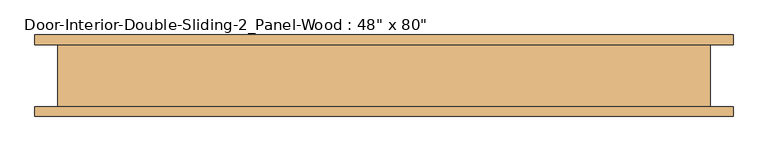
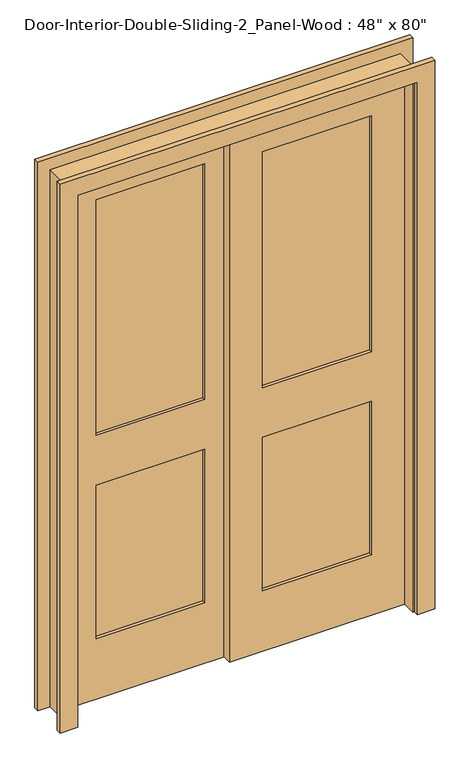
"""IFC4 building model written with IfcOpenShell, lengths in millimetres: door geometry."""

import ifcopenshell
import ifcopenshell.guid

model = None  # the IFC model being written
_history = None  # IfcOwnerHistory: only IFC2X3 demands one
_inside = {}  # id of a spatial element -> (the spatial element, [elements in it])
_under = {}  # id of a project, library or spatial element -> (it, [spatial elements below it])
_declared = {}  # id of a project -> (the project, [libraries it declares])
_typed = {}  # id of a type object -> (the type object, [elements of that type])
_made_of = {}  # id of a material, layer set ... -> (it, [elements and type objects made of it])


def new_model(schema):
    """Start an empty IFC model of exactly this schema.

    Asked for "IFC4X3", IfcOpenShell would pick the latest addendum, in which some entities
    have other attributes; the version numbers below select the first issue.
    IFC2X3 requires an IfcOwnerHistory on every rooted entity: one is made here for all.
    """
    global model, _history
    if schema == "IFC4X3":
        model = ifcopenshell.file(schema_version=(4, 3, 0, 0))
    else:
        model = ifcopenshell.file(schema=schema)
    _inside.clear()
    _under.clear()
    _declared.clear()
    _typed.clear()
    _made_of.clear()
    _history = None
    if model.schema == "IFC2X3":
        org = make("IfcOrganization", Name="unknown")
        user = make(
            "IfcPersonAndOrganization",
            ThePerson=make("IfcPerson", FamilyName="unknown"),
            TheOrganization=org,
        )
        app = make(
            "IfcApplication",
            ApplicationDeveloper=org,
            Version="unknown",
            ApplicationFullName="unknown",
            ApplicationIdentifier="unknown",
        )
        _history = make(
            "IfcOwnerHistory",
            OwningUser=user,
            OwningApplication=app,
            ChangeAction="ADDED",
            CreationDate=0,
        )
    return model


def make(cls, **values):
    """One entity of the class cls with the attributes given. An attribute that is None is left unset."""
    return model.create_entity(
        cls, **{name: value for name, value in values.items() if value is not None}
    )


def rooted(cls, **values):
    """An entity with a GlobalId (a new one), such as an element, a storey or a relation."""
    return make(cls, GlobalId=ifcopenshell.guid.new(), OwnerHistory=_history, **values)


def si_unit(unit_type, name, prefix=None):
    """IfcSIUnit, for example si_unit("LENGTHUNIT", "METRE", prefix="MILLI")."""
    return make("IfcSIUnit", UnitType=unit_type, Prefix=prefix, Name=name)


def assignment(units):
    """IfcUnitAssignment: the units of a project."""
    return None if units is None else make("IfcUnitAssignment", Units=units)


def point(xyz):
    """IfcCartesianPoint."""
    return None if xyz is None else make("IfcCartesianPoint", Coordinates=xyz)


def direction(xyz):
    """IfcDirection."""
    return None if xyz is None else make("IfcDirection", DirectionRatios=xyz)


def frame(location, z_axis=None, x_axis=None):
    """IfcAxis2Placement3D, a coordinate frame: its origin and axes. An axis left out is left unset."""
    return make(
        "IfcAxis2Placement3D",
        Location=point(location),
        Axis=direction(z_axis),
        RefDirection=direction(x_axis),
    )


def origin():
    """The frame at (0, 0, 0) with its axes left unset."""
    return frame((0.0, 0.0, 0.0))


def place(relative_to, where):
    """IfcLocalPlacement: puts the frame where relative to a parent placement (None: the world)."""
    return make(
        "IfcLocalPlacement", PlacementRelTo=relative_to, RelativePlacement=where
    )


def context(
    kind, dimensions, precision=None, world=None, true_north=None, identifier=None
):
    """IfcGeometricRepresentationContext, for example the 3D "Model" context."""
    return make(
        "IfcGeometricRepresentationContext",
        ContextIdentifier=identifier,
        ContextType=kind,
        CoordinateSpaceDimension=dimensions,
        Precision=precision,
        WorldCoordinateSystem=world,
        TrueNorth=true_north,
    )


def project(units=None, contexts=None):
    """IfcProject with its units and contexts."""
    return rooted(
        "IfcProject",
        Name="project",
        RepresentationContexts=contexts,
        UnitsInContext=assignment(units),
    )


def spatial(cls, under=None, at=None, **own):
    """A site, building, storey or space (cls), placed at a placement, below another one or the project."""
    s = rooted(cls, ObjectPlacement=at, **own)
    if under is not None:
        _under.setdefault(under.id(), (under, []))[1].append(s)
    return s


def polyline(points):
    """IfcPolyline through the points."""
    return make("IfcPolyline", Points=[point(p) for p in points])


def outline(outer, holes=None, kind="AREA"):
    """IfcArbitraryClosedProfileDef: a profile drawn as a closed curve; with holes, ...WithVoids."""
    if holes is None:
        return make("IfcArbitraryClosedProfileDef", ProfileType=kind, OuterCurve=outer)
    return make(
        "IfcArbitraryProfileDefWithVoids",
        ProfileType=kind,
        OuterCurve=outer,
        InnerCurves=holes,
    )


def extrude(swept, where, along, depth):
    """IfcExtrudedAreaSolid: the profile swept, set in the frame where, extruded along a direction by depth."""
    return make(
        "IfcExtrudedAreaSolid",
        SweptArea=swept,
        Position=where,
        ExtrudedDirection=direction(along),
        Depth=depth,
    )


def shape(context_of_items, identifier, shape_type, items):
    """IfcShapeRepresentation: the items that make up one representation, for example the "Body"."""
    return make(
        "IfcShapeRepresentation",
        ContextOfItems=context_of_items,
        RepresentationIdentifier=identifier,
        RepresentationType=shape_type,
        Items=items,
    )


def source(mapping_origin, context_of_items, identifier, shape_type, items):
    """IfcRepresentationMap: a shape defined once, which mapped items show again and again."""
    return make(
        "IfcRepresentationMap",
        MappingOrigin=mapping_origin,
        MappedRepresentation=shape(context_of_items, identifier, shape_type, items),
    )


def transform(
    local_origin,
    x_axis=None,
    y_axis=None,
    z_axis=None,
    scale=None,
    scale2=None,
    scale3=None,
    uniform=True,
):
    """IfcCartesianTransformationOperator3D, or its non-uniform kind. x_axis, y_axis, z_axis: its Axis1, 2, 3."""
    if uniform:
        return make(
            "IfcCartesianTransformationOperator3D",
            Axis1=direction(x_axis),
            Axis2=direction(y_axis),
            LocalOrigin=point(local_origin),
            Scale=scale,
            Axis3=direction(z_axis),
        )
    return make(
        "IfcCartesianTransformationOperator3DnonUniform",
        Axis1=direction(x_axis),
        Axis2=direction(y_axis),
        LocalOrigin=point(local_origin),
        Scale=scale,
        Axis3=direction(z_axis),
        Scale2=scale2,
        Scale3=scale3,
    )


def mapped(mapping_source, mapping_target):
    """IfcMappedItem: shows the shape of a source again, moved by a transform."""
    return make(
        "IfcMappedItem", MappingSource=mapping_source, MappingTarget=mapping_target
    )


def made_of(thing, what):
    """Note that an element or type object is made of a material, layer set ...; save() writes the relation."""
    if what is not None:
        _made_of.setdefault(what.id(), (what, []))[1].append(thing)
    return thing


def element(
    cls,
    number,
    at=None,
    inside=None,
    cuts=None,
    type_object=None,
    material=None,
    context=None,
    identifier="Body",
    shape_type=None,
    held_by="IfcProductDefinitionShape",
    body=None,
    shapes=None,
    **own,
):
    """One element of the class cls, such as IfcWall. Its Tag is "e" and its number.

    at: its placement. inside: the storey or other place that contains it. cuts: it is an
    opening in that element (IfcRelVoidsElement). A single representation is given by context,
    identifier, shape_type and body (its items); several are given by shapes. held_by: the class
    of the entity that holds the representations. save() writes the other relations.
    """
    e = rooted(cls, Tag="e%d" % number, ObjectPlacement=at, **own)
    if body is not None:
        shapes = [shape(context, identifier, shape_type, body)]
    if shapes is not None:
        e.Representation = make(held_by, Representations=shapes)
    if inside is not None:
        _inside.setdefault(inside.id(), (inside, []))[1].append(e)
    if cuts is not None:
        rooted(
            "IfcRelVoidsElement", RelatingBuildingElement=cuts, RelatedOpeningElement=e
        )
    if type_object is not None:
        _typed.setdefault(type_object.id(), (type_object, []))[1].append(e)
    return made_of(e, material)


def aggregate(whole, parts):
    """IfcRelAggregates: a whole, such as a stair, and the parts it consists of."""
    return rooted("IfcRelAggregates", RelatingObject=whole, RelatedObjects=parts)


def save(model, path):
    """Write the relations noted so far, then the file.

    IfcRelAggregates (storeys below a building ...), IfcRelContainedInSpatialStructure (elements
    in a storey), IfcRelDefinesByType, IfcRelAssociatesMaterial and IfcRelDeclares: one each for
    every whole, place, type object, material and project.
    """
    for whole, parts in _under.values():
        aggregate(whole, parts)
    for where, things in _inside.values():
        rooted(
            "IfcRelContainedInSpatialStructure",
            RelatedElements=things,
            RelatingStructure=where,
        )
    for kind, things in _typed.values():
        rooted("IfcRelDefinesByType", RelatedObjects=things, RelatingType=kind)
    for what, things in _made_of.values():
        rooted("IfcRelAssociatesMaterial", RelatedObjects=things, RelatingMaterial=what)
    for by, libraries in _declared.values():
        rooted("IfcRelDeclares", RelatingContext=by, RelatedDefinitions=libraries)
    model.write(path)


def door_5e6fa93e(model_context):
    return source(origin(), model_context, "Body", "SweptSolid", [
        extrude(outline(polyline([(488.95, -1.0583333), (95.25, -1.0583333), (95.25, 10.5833333), (488.95, 10.5833333), (488.95, -1.0583333)])), frame((0.0, 0.0, 1009.65), z_axis=(0.0, 0.0, 1.0), x_axis=(1.0, 0.0, 0.0)), (0.0, 0.0, 1.0), 903.2875),
        extrude(outline(polyline([(488.95, -1.0583333), (95.25, -1.0583333), (95.25, 10.5833333), (488.95, 10.5833333), (488.95, -1.0583333)])), frame((0.0, 0.0, 231.775), z_axis=(0.0, 0.0, 1.0), x_axis=(1.0, 0.0, 0.0)), (0.0, 0.0, 1.0), 587.375),
        extrude(outline(polyline([(2032.0, -25.4), (0.0, -25.4), (0.0, 609.6), (2032.0, 609.6), (2032.0, -25.4)]), holes=[polyline([(1912.9375, 95.25), (1912.9375, 488.95), (1009.65, 488.95), (1009.65, 95.25), (1912.9375, 95.25)]), polyline([(819.15, 95.25), (819.15, 488.95), (231.775, 488.95), (231.775, 95.25), (819.15, 95.25)])]), frame((0.0, -12.7, 0.0), z_axis=(0.0, 1.0, 0.0), x_axis=(0.0, 0.0, 1.0)), (0.0, 0.0, 1.0), 34.925),
        extrude(outline(polyline([(-95.25, 33.8666667), (-488.95, 33.8666667), (-488.95, 45.5083333), (-95.25, 45.5083333), (-95.25, 33.8666667)])), frame((0.0, 0.0, 1009.65), z_axis=(0.0, 0.0, 1.0), x_axis=(1.0, 0.0, 0.0)), (0.0, 0.0, 1.0), 903.2875),
        extrude(outline(polyline([(-95.25, 33.8666667), (-488.95, 33.8666667), (-488.95, 45.5083333), (-95.25, 45.5083333), (-95.25, 33.8666667)])), frame((0.0, 0.0, 231.775), z_axis=(0.0, 0.0, 1.0), x_axis=(1.0, 0.0, 0.0)), (0.0, 0.0, 1.0), 587.375),
        extrude(outline(polyline([(2032.0, -609.6), (0.0, -609.6), (0.0, 25.4), (2032.0, 25.4), (2032.0, -609.6)]), holes=[polyline([(1912.9375, -488.95), (1912.9375, -95.25), (1009.65, -95.25), (1009.65, -488.95), (1912.9375, -488.95)]), polyline([(819.15, -488.95), (819.15, -95.25), (231.775, -95.25), (231.775, -488.95), (819.15, -488.95)])]), frame((0.0, 22.225, 0.0), z_axis=(0.0, 1.0, 0.0), x_axis=(0.0, 0.0, 1.0)), (0.0, 0.0, 1.0), 34.925),
        extrude(outline(polyline([(0.0, 609.6), (0.0, 635.0), (2057.4, 635.0), (2057.4, -635.0), (0.0, -635.0), (0.0, -609.6), (2032.0, -609.6), (2032.0, 609.6), (0.0, 609.6)])), frame((0.0, -63.5, 0.0), z_axis=(0.0, 1.0, 0.0), x_axis=(0.0, 0.0, 1.0)), (0.0, 0.0, 1.0), 120.65),
        extrude(outline(polyline([(0.0, 615.95), (0.0, 679.45), (2101.85, 679.45), (2101.85, -679.45), (0.0, -679.45), (0.0, -615.95), (2038.35, -615.95), (2038.35, 615.95), (0.0, 615.95)])), frame((0.0, -82.55, 0.0), z_axis=(0.0, 1.0, 0.0), x_axis=(0.0, 0.0, 1.0)), (0.0, 0.0, 1.0), 19.05),
        extrude(outline(polyline([(0.0, 615.95), (0.0, 679.45), (2101.85, 679.45), (2101.85, -679.45), (0.0, -679.45), (0.0, -615.95), (2038.35, -615.95), (2038.35, 615.95), (0.0, 615.95)])), frame((0.0, 57.15, 0.0), z_axis=(0.0, 1.0, 0.0), x_axis=(0.0, 0.0, 1.0)), (0.0, 0.0, 1.0), 19.05),
    ])


if __name__ == "__main__":
    model = new_model("IFC4")
    model_context = context("Model", 3, world=origin())
    ifc_project = project(units=[si_unit("LENGTHUNIT", "METRE", prefix="MILLI")], contexts=[model_context])
    site = spatial("IfcSite", under=ifc_project)
    building = spatial("IfcBuilding", under=site)
    placement = place(None, origin())
    door_shape = door_5e6fa93e(model_context)
    element("IfcDoor", 1, ObjectType="Door-Interior-Double-Sliding-2_Panel-Wood : 48\" x 80\"", at=placement, inside=building, context=model_context, shape_type="MappedRepresentation", body=[
        mapped(door_shape, transform((0.0, 0.0, 0.0), x_axis=(1.0, 0.0, 0.0), y_axis=(0.0, 1.0, 0.0), z_axis=(0.0, 0.0, 1.0))),
    ])
    save(model, "model.ifc")

# Revit data of these elements
# Type "Door-Interior-Double-Sliding-2_Panel-Wood : 48\" x 80\""
#   Type Mark = "22"
#   Assembly Code = "C1020300"
#   Analytic Construction = "Wooden"
#   Top Rail = 0' - 4 11/16"
#   Thickness = 0' - 1 3/8"
#   Thermal Resistance (R) = 2.5876 (h·ft²·°F)/BTU
#   Stiles = 0' - 4 3/4"
#   Rough Width = 4' - 2"
#   Rough Height = 6' - 9"
#   Lock Rail = 0' - 7 1/2"
#   Height = 6' - 8"
#   Width = 4' - 0"
#   Heat Transfer Coefficient (U) = 0.3865 BTU/(h·ft²·°F)
#   Bottom Rail = 0' - 9 1/8"
#   Trim Material = Cherry
#   Panel Material = Cherry
#   Frame Material = Cherry
#   Visual Light Transmittance = 0
#   Solar Heat Gain Coefficient = 0
#   Wall Closure = (empty or 0)
#   Function = (empty or 0)
# Element 1 (IfcDoor, "Door-Interior-Double-Sliding-2_Panel-Wood : 48\" x 80\"")
#   Materials on its faces: "Cherry"
# Materials
#   "Cherry": class "Wood", colour RGB 226 177 128, transparency 0, Description = "Prunus Serotina", Cost = 0
